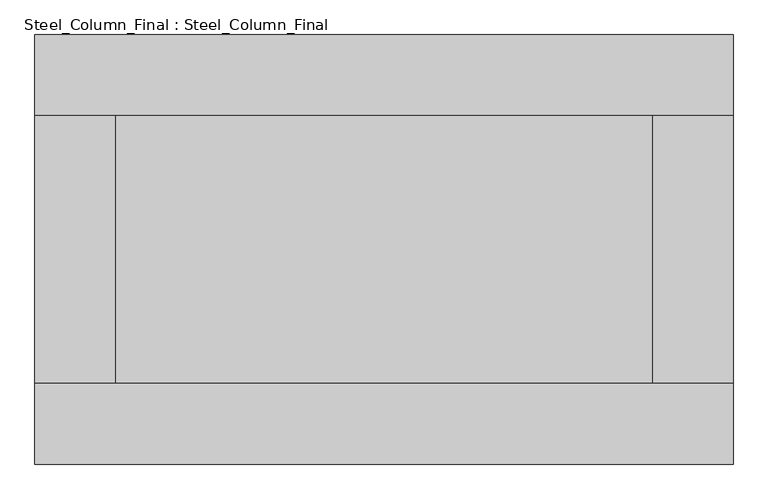
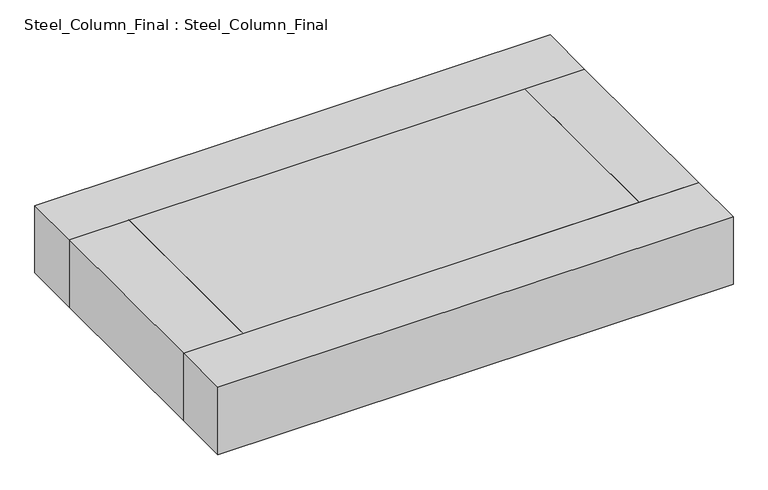
"""IFC4 building model written with IfcOpenShell, lengths in millimetres: proxy geometry, Steel_Column_Final : Steel_Column_Final."""

from ifc_helpers import new_model, si_unit, frame, origin, place, context, project, spatial, polyline, outline, extrude, source, transform, mapped, element, save


def steel_column_final_steel_column_final_81e61526(model_context):
    return source(origin(), model_context, "Body", "SweptSolid", [
        extrude(outline(polyline([(6500.0, 2500.0), (-6500.0, 2500.0), (-6500.0, 4000.0), (6500.0, 4000.0), (6500.0, 2500.0)])), frame((0.0, 0.0, 104400.0), z_axis=(0.0, 0.0, 1.0), x_axis=(1.0, 0.0, 0.0)), (0.0, 0.0, 1.0), 1800.0),
        extrude(outline(polyline([(-6500.0, -2500.0), (6500.0, -2500.0), (6500.0, -4000.0), (-6500.0, -4000.0), (-6500.0, -2500.0)])), frame((0.0, 0.0, 104400.0), z_axis=(0.0, 0.0, 1.0), x_axis=(1.0, 0.0, 0.0)), (0.0, 0.0, 1.0), 1800.0),
        extrude(outline(polyline([(5000.0, -2500.0), (5000.0, 2500.0), (6500.0, 2500.0), (6500.0, -2500.0), (5000.0, -2500.0)])), frame((0.0, 0.0, 104400.0), z_axis=(0.0, 0.0, 1.0), x_axis=(1.0, 0.0, 0.0)), (0.0, 0.0, 1.0), 1800.0),
        extrude(outline(polyline([(-5000.0, 2500.0), (-5000.0, -2500.0), (-6500.0, -2500.0), (-6500.0, 2500.0), (-5000.0, 2500.0)])), frame((0.0, 0.0, 104400.0), z_axis=(0.0, 0.0, 1.0), x_axis=(1.0, 0.0, 0.0)), (0.0, 0.0, 1.0), 1800.0),
        extrude(outline(polyline([(-5000.0, -2500.0), (-5000.0, 2500.0), (5000.0, 2500.0), (5000.0, -2500.0), (-5000.0, -2500.0)])), frame((0.0, 0.0, 104400.0), z_axis=(0.0, 0.0, 1.0), x_axis=(1.0, 0.0, 0.0)), (0.0, 0.0, 1.0), 1800.0),
    ])


if __name__ == "__main__":
    model = new_model("IFC4")
    model_context = context("Model", 3, world=origin())
    ifc_project = project(units=[si_unit("LENGTHUNIT", "METRE", prefix="MILLI")], contexts=[model_context])
    site = spatial("IfcSite", under=ifc_project)
    building = spatial("IfcBuilding", under=site)
    placement = place(None, origin())
    steel_column_final_steel_column_final_shape = steel_column_final_steel_column_final_81e61526(model_context)
    element("IfcBuildingElementProxy", 1, Name="Steel_Column_Final : Steel_Column_Final", ObjectType="Steel_Column_Final : Steel_Column_Final", at=placement, inside=building, context=model_context, shape_type="MappedRepresentation", body=[
        mapped(steel_column_final_steel_column_final_shape, transform((0.0, 0.0, 0.0), x_axis=(1.0, 0.0, 0.0), y_axis=(0.0, 1.0, 0.0), z_axis=(0.0, 0.0, 1.0))),
    ])
    save(model, "model.ifc")

# Revit data of these elements
# Type "Steel_Column_Final : Steel_Column_Final"
#   Top Width [instance default] = 5000 mm
#   Top Length = 10000 mm
#   Length = 21000 mm
#   Height [instance default] = 50000 mm
#   Bottom Width [instance default] = 5000 mm
#   Default Elevation = 0
# Element 1 (IfcBuildingElementProxy, "Steel_Column_Final : Steel_Column_Final")
#   Height = 104400 mm
